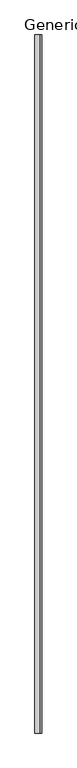
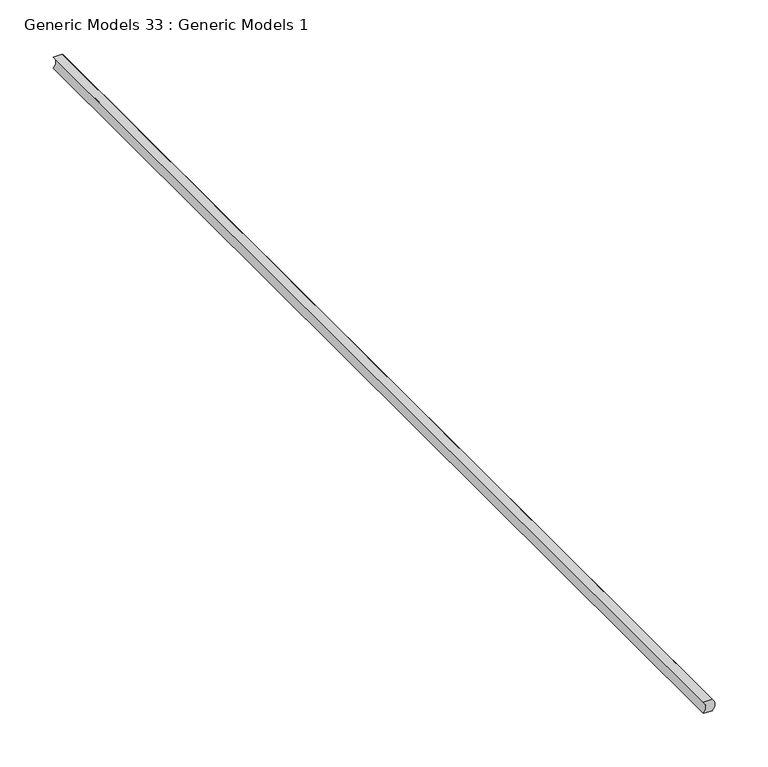
"""IFC4 building model written with IfcOpenShell, lengths in millimetres: proxy geometry, Generic Models 33 : Generic Models 1."""

import ifcopenshell
import ifcopenshell.guid

model = None  # the IFC model being written
_history = None  # IfcOwnerHistory: only IFC2X3 demands one
_inside = {}  # id of a spatial element -> (the spatial element, [elements in it])
_under = {}  # id of a project, library or spatial element -> (it, [spatial elements below it])
_declared = {}  # id of a project -> (the project, [libraries it declares])
_typed = {}  # id of a type object -> (the type object, [elements of that type])
_made_of = {}  # id of a material, layer set ... -> (it, [elements and type objects made of it])


def new_model(schema):
    """Start an empty IFC model of exactly this schema.

    Asked for "IFC4X3", IfcOpenShell would pick the latest addendum, in which some entities
    have other attributes; the version numbers below select the first issue.
    IFC2X3 requires an IfcOwnerHistory on every rooted entity: one is made here for all.
    """
    global model, _history
    if schema == "IFC4X3":
        model = ifcopenshell.file(schema_version=(4, 3, 0, 0))
    else:
        model = ifcopenshell.file(schema=schema)
    _inside.clear()
    _under.clear()
    _declared.clear()
    _typed.clear()
    _made_of.clear()
    _history = None
    if model.schema == "IFC2X3":
        org = make("IfcOrganization", Name="unknown")
        user = make(
            "IfcPersonAndOrganization",
            ThePerson=make("IfcPerson", FamilyName="unknown"),
            TheOrganization=org,
        )
        app = make(
            "IfcApplication",
            ApplicationDeveloper=org,
            Version="unknown",
            ApplicationFullName="unknown",
            ApplicationIdentifier="unknown",
        )
        _history = make(
            "IfcOwnerHistory",
            OwningUser=user,
            OwningApplication=app,
            ChangeAction="ADDED",
            CreationDate=0,
        )
    return model


def make(cls, **values):
    """One entity of the class cls with the attributes given. An attribute that is None is left unset."""
    return model.create_entity(
        cls, **{name: value for name, value in values.items() if value is not None}
    )


def rooted(cls, **values):
    """An entity with a GlobalId (a new one), such as an element, a storey or a relation."""
    return make(cls, GlobalId=ifcopenshell.guid.new(), OwnerHistory=_history, **values)


def si_unit(unit_type, name, prefix=None):
    """IfcSIUnit, for example si_unit("LENGTHUNIT", "METRE", prefix="MILLI")."""
    return make("IfcSIUnit", UnitType=unit_type, Prefix=prefix, Name=name)


def assignment(units):
    """IfcUnitAssignment: the units of a project."""
    return None if units is None else make("IfcUnitAssignment", Units=units)


def point(xyz):
    """IfcCartesianPoint."""
    return None if xyz is None else make("IfcCartesianPoint", Coordinates=xyz)


def direction(xyz):
    """IfcDirection."""
    return None if xyz is None else make("IfcDirection", DirectionRatios=xyz)


def frame(location, z_axis=None, x_axis=None):
    """IfcAxis2Placement3D, a coordinate frame: its origin and axes. An axis left out is left unset."""
    return make(
        "IfcAxis2Placement3D",
        Location=point(location),
        Axis=direction(z_axis),
        RefDirection=direction(x_axis),
    )


def frame_2d(location, x_axis=None):
    """IfcAxis2Placement2D, a coordinate frame in the plane: its origin and x axis."""
    return make(
        "IfcAxis2Placement2D", Location=point(location), RefDirection=direction(x_axis)
    )


def origin():
    """The frame at (0, 0, 0) with its axes left unset."""
    return frame((0.0, 0.0, 0.0))


def place(relative_to, where):
    """IfcLocalPlacement: puts the frame where relative to a parent placement (None: the world)."""
    return make(
        "IfcLocalPlacement", PlacementRelTo=relative_to, RelativePlacement=where
    )


def context(
    kind, dimensions, precision=None, world=None, true_north=None, identifier=None
):
    """IfcGeometricRepresentationContext, for example the 3D "Model" context."""
    return make(
        "IfcGeometricRepresentationContext",
        ContextIdentifier=identifier,
        ContextType=kind,
        CoordinateSpaceDimension=dimensions,
        Precision=precision,
        WorldCoordinateSystem=world,
        TrueNorth=true_north,
    )


def project(units=None, contexts=None):
    """IfcProject with its units and contexts."""
    return rooted(
        "IfcProject",
        Name="project",
        RepresentationContexts=contexts,
        UnitsInContext=assignment(units),
    )


def spatial(cls, under=None, at=None, **own):
    """A site, building, storey or space (cls), placed at a placement, below another one or the project."""
    s = rooted(cls, ObjectPlacement=at, **own)
    if under is not None:
        _under.setdefault(under.id(), (under, []))[1].append(s)
    return s


def polyline(points):
    """IfcPolyline through the points."""
    return make("IfcPolyline", Points=[point(p) for p in points])


def circle_curve(where, radius):
    """IfcCircle in the frame where."""
    return make("IfcCircle", Position=where, Radius=radius)


def trimmed(basis, trim1, trim2, sense, master):
    """IfcTrimmedCurve: the piece of a basis curve between two trims."""
    return make(
        "IfcTrimmedCurve",
        BasisCurve=basis,
        Trim1=trim1,
        Trim2=trim2,
        SenseAgreement=sense,
        MasterRepresentation=master,
    )


def segment(curve, same_sense, transition):
    """IfcCompositeCurveSegment."""
    return make(
        "IfcCompositeCurveSegment",
        Transition=transition,
        SameSense=same_sense,
        ParentCurve=curve,
    )


def composite_curve(segments, self_intersect=None):
    """IfcCompositeCurve: segments joined end to end."""
    return make("IfcCompositeCurve", Segments=segments, SelfIntersect=self_intersect)


def outline(outer, holes=None, kind="AREA"):
    """IfcArbitraryClosedProfileDef: a profile drawn as a closed curve; with holes, ...WithVoids."""
    if holes is None:
        return make("IfcArbitraryClosedProfileDef", ProfileType=kind, OuterCurve=outer)
    return make(
        "IfcArbitraryProfileDefWithVoids",
        ProfileType=kind,
        OuterCurve=outer,
        InnerCurves=holes,
    )


def extrude(swept, where, along, depth):
    """IfcExtrudedAreaSolid: the profile swept, set in the frame where, extruded along a direction by depth."""
    return make(
        "IfcExtrudedAreaSolid",
        SweptArea=swept,
        Position=where,
        ExtrudedDirection=direction(along),
        Depth=depth,
    )


def shape(context_of_items, identifier, shape_type, items):
    """IfcShapeRepresentation: the items that make up one representation, for example the "Body"."""
    return make(
        "IfcShapeRepresentation",
        ContextOfItems=context_of_items,
        RepresentationIdentifier=identifier,
        RepresentationType=shape_type,
        Items=items,
    )


def source(mapping_origin, context_of_items, identifier, shape_type, items):
    """IfcRepresentationMap: a shape defined once, which mapped items show again and again."""
    return make(
        "IfcRepresentationMap",
        MappingOrigin=mapping_origin,
        MappedRepresentation=shape(context_of_items, identifier, shape_type, items),
    )


def transform(
    local_origin,
    x_axis=None,
    y_axis=None,
    z_axis=None,
    scale=None,
    scale2=None,
    scale3=None,
    uniform=True,
):
    """IfcCartesianTransformationOperator3D, or its non-uniform kind. x_axis, y_axis, z_axis: its Axis1, 2, 3."""
    if uniform:
        return make(
            "IfcCartesianTransformationOperator3D",
            Axis1=direction(x_axis),
            Axis2=direction(y_axis),
            LocalOrigin=point(local_origin),
            Scale=scale,
            Axis3=direction(z_axis),
        )
    return make(
        "IfcCartesianTransformationOperator3DnonUniform",
        Axis1=direction(x_axis),
        Axis2=direction(y_axis),
        LocalOrigin=point(local_origin),
        Scale=scale,
        Axis3=direction(z_axis),
        Scale2=scale2,
        Scale3=scale3,
    )


def mapped(mapping_source, mapping_target):
    """IfcMappedItem: shows the shape of a source again, moved by a transform."""
    return make(
        "IfcMappedItem", MappingSource=mapping_source, MappingTarget=mapping_target
    )


def made_of(thing, what):
    """Note that an element or type object is made of a material, layer set ...; save() writes the relation."""
    if what is not None:
        _made_of.setdefault(what.id(), (what, []))[1].append(thing)
    return thing


def element(
    cls,
    number,
    at=None,
    inside=None,
    cuts=None,
    type_object=None,
    material=None,
    context=None,
    identifier="Body",
    shape_type=None,
    held_by="IfcProductDefinitionShape",
    body=None,
    shapes=None,
    **own,
):
    """One element of the class cls, such as IfcWall. Its Tag is "e" and its number.

    at: its placement. inside: the storey or other place that contains it. cuts: it is an
    opening in that element (IfcRelVoidsElement). A single representation is given by context,
    identifier, shape_type and body (its items); several are given by shapes. held_by: the class
    of the entity that holds the representations. save() writes the other relations.
    """
    e = rooted(cls, Tag="e%d" % number, ObjectPlacement=at, **own)
    if body is not None:
        shapes = [shape(context, identifier, shape_type, body)]
    if shapes is not None:
        e.Representation = make(held_by, Representations=shapes)
    if inside is not None:
        _inside.setdefault(inside.id(), (inside, []))[1].append(e)
    if cuts is not None:
        rooted(
            "IfcRelVoidsElement", RelatingBuildingElement=cuts, RelatedOpeningElement=e
        )
    if type_object is not None:
        _typed.setdefault(type_object.id(), (type_object, []))[1].append(e)
    return made_of(e, material)


def aggregate(whole, parts):
    """IfcRelAggregates: a whole, such as a stair, and the parts it consists of."""
    return rooted("IfcRelAggregates", RelatingObject=whole, RelatedObjects=parts)


def save(model, path):
    """Write the relations noted so far, then the file.

    IfcRelAggregates (storeys below a building ...), IfcRelContainedInSpatialStructure (elements
    in a storey), IfcRelDefinesByType, IfcRelAssociatesMaterial and IfcRelDeclares: one each for
    every whole, place, type object, material and project.
    """
    for whole, parts in _under.values():
        aggregate(whole, parts)
    for where, things in _inside.values():
        rooted(
            "IfcRelContainedInSpatialStructure",
            RelatedElements=things,
            RelatingStructure=where,
        )
    for kind, things in _typed.values():
        rooted("IfcRelDefinesByType", RelatedObjects=things, RelatingType=kind)
    for what, things in _made_of.values():
        rooted("IfcRelAssociatesMaterial", RelatedObjects=things, RelatingMaterial=what)
    for by, libraries in _declared.values():
        rooted("IfcRelDeclares", RelatingContext=by, RelatedDefinitions=libraries)
    model.write(path)


def generic_models_33_generic_models_1_084f7e48(model_context):
    return source(origin(), model_context, "Body", "SweptSolid", [
        extrude(outline(composite_curve([segment(polyline([(2438.4, 48444.15), (2438.4, 48453.675)]), True, "CONTINUOUS"), segment(trimmed(circle_curve(frame_2d((2444.75, 48447.845519)), 8.620055), [point((2438.4, 48453.675))], [point((2451.1, 48453.675))], False, "CARTESIAN"), True, "CONTINUOUS"), segment(polyline([(2451.1, 48453.675), (2451.1, 48444.15)]), True, "CONTINUOUS"), segment(trimmed(circle_curve(frame_2d((2444.75, 48438.320519)), 8.620055), [point((2451.1, 48444.15))], [point((2438.4, 48444.15))], True, "CARTESIAN"), True, "CONTINUOUS")], self_intersect=False)), frame((0.0, 0.0, 0.0), z_axis=(0.0, 1.0, 0.0), x_axis=(0.0, 0.0, 1.0)), (0.0, 0.0, 1.0), 1219.2),
    ])


if __name__ == "__main__":
    model = new_model("IFC4")
    model_context = context("Model", 3, world=origin())
    ifc_project = project(units=[si_unit("LENGTHUNIT", "METRE", prefix="MILLI")], contexts=[model_context])
    site = spatial("IfcSite", under=ifc_project)
    building = spatial("IfcBuilding", under=site)
    placement = place(None, origin())
    generic_models_33_generic_models_1_shape = generic_models_33_generic_models_1_084f7e48(model_context)
    element("IfcBuildingElementProxy", 1, Name="Generic Models 33 : Generic Models 1", ObjectType="Generic Models 33 : Generic Models 1", at=placement, inside=building, context=model_context, shape_type="MappedRepresentation", body=[
        mapped(generic_models_33_generic_models_1_shape, transform((0.0, 0.0, 0.0), x_axis=(1.0, 0.0, 0.0), y_axis=(0.0, 1.0, 0.0), z_axis=(0.0, 0.0, 1.0))),
    ])
    save(model, "model.ifc")

# Revit data of these elements
# Project information
#   Project Issue Date = "Issue Date"
#   Project Status = "Project Status"
#   Client Name = "Owner"
#   Project Address = "Enter address here"
#   Project Name = "Haubenschild World Headquarters"
#   Project Number = "Project Number"
# Element 1 (IfcBuildingElementProxy, "Generic Models 33 : Generic Models 1")
#   Materials on its faces: "ACOUSTICAL SEALANT"
# Materials
#   "ACOUSTICAL SEALANT": class "Unassigned", colour RGB 120 120 120, transparency 0, Cost = 0
